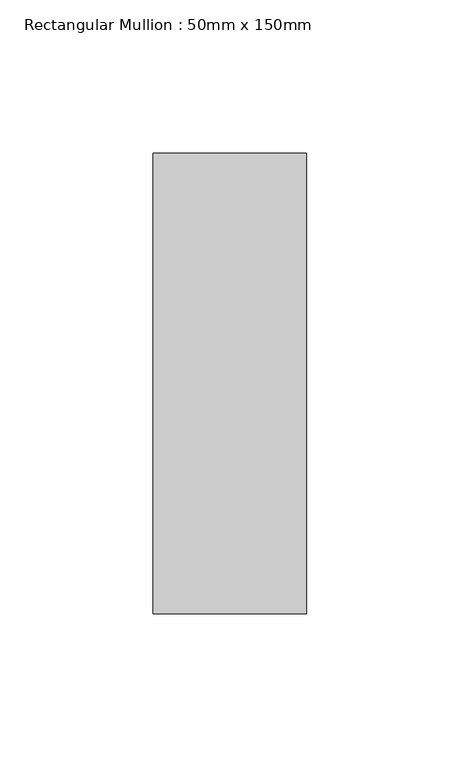
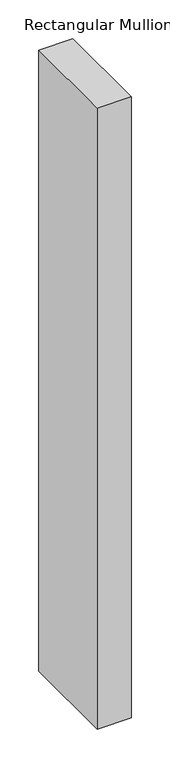
"""IFC4 building model written with IfcOpenShell, lengths in millimetres: member geometry, Rectangular Mullion : 50mm x 150mm."""

from ifc_helpers import new_model, si_unit, frame, origin, place, context, project, spatial, polyline, outline, extrude, source, transform, mapped, element, save


def rectangular_mullion_50mm_x_150mm_20c262b5(model_context):
    return source(origin(), model_context, "Body", "SweptSolid", [
        extrude(outline(polyline([(0.0, 75.0), (0.0, -75.0), (-50.0, -75.0), (-50.0, 75.0), (0.0, 75.0)])), frame((0.0, 0.0, -973.5877237), z_axis=(0.0, 0.0, 1.0), x_axis=(1.0, 0.0, 0.0)), (0.0, 0.0, 1.0), 973.5877237),
    ])


if __name__ == "__main__":
    model = new_model("IFC4")
    model_context = context("Model", 3, world=origin())
    ifc_project = project(units=[si_unit("LENGTHUNIT", "METRE", prefix="MILLI")], contexts=[model_context])
    site = spatial("IfcSite", under=ifc_project)
    building = spatial("IfcBuilding", under=site)
    placement = place(None, origin())
    rectangular_mullion_50mm_x_150mm_shape = rectangular_mullion_50mm_x_150mm_20c262b5(model_context)
    element("IfcMember", 1, ObjectType="Rectangular Mullion : 50mm x 150mm", at=placement, inside=building, context=model_context, shape_type="MappedRepresentation", body=[
        mapped(rectangular_mullion_50mm_x_150mm_shape, transform((0.0, 0.0, 0.0), x_axis=(1.0, 0.0, 0.0), y_axis=(0.0, 1.0, 0.0), z_axis=(0.0, 0.0, 1.0))),
    ])
    save(model, "model.ifc")

# Revit data of these elements
# Type "Rectangular Mullion : 50mm x 150mm"
#   built-in parameter 1007304 = 0.492126 (stored number, unit not read)
#   built-in parameter 1007301 = 0.082021 (stored number, unit not read)
#   built-in parameter 1007300 = 0.082021 (stored number, unit not read)
# Element 1 (IfcMember, "Rectangular Mullion : 50mm x 150mm")
#   Materials on its faces: "Aluminum"
# Materials
#   "Aluminum": class "Metal", colour RGB 247 247 247, transparency 0, Description = "Aluminum 6061", Cost = 0
